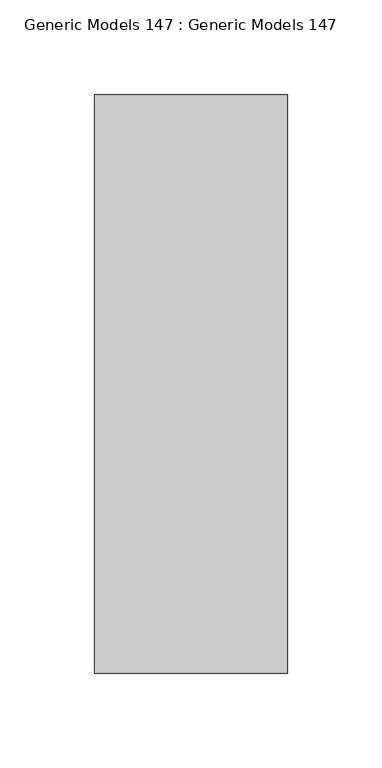
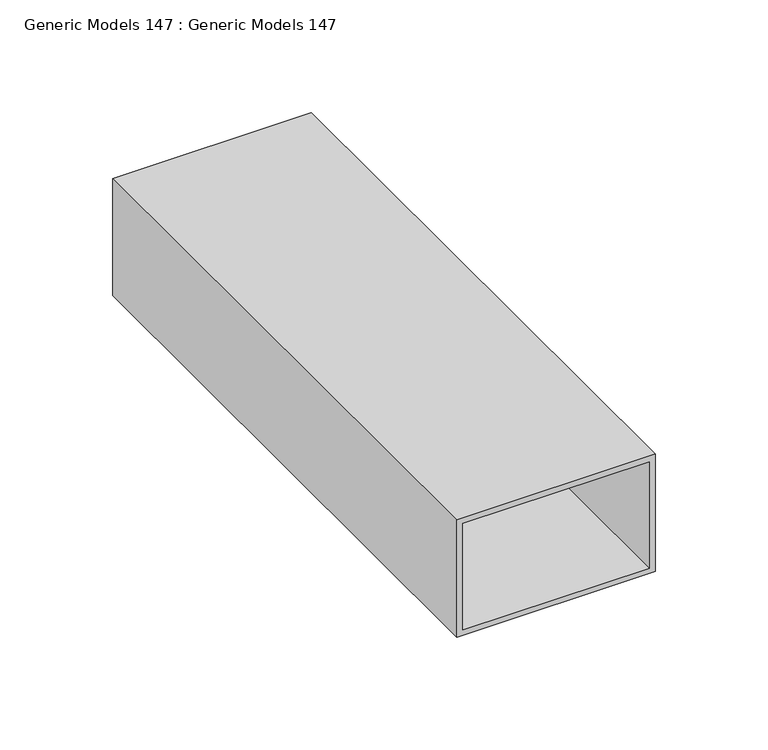
"""IFC4 building model written with IfcOpenShell, lengths in millimetres: proxy geometry, Generic Models 147 : Generic Models 147."""

from ifc_helpers import new_model, si_unit, frame, origin, place, context, project, spatial, polyline, outline, extrude, source, transform, mapped, element, save


def generic_models_147_generic_models_147_e6257d2f(model_context):
    return source(origin(), model_context, "Body", "SweptSolid", [
        extrude(outline(polyline([(126263.146, 4942.0939304), (126263.146, 4840.4939304), (126199.646, 4840.4939304), (126199.646, 4942.0939304), (126263.146, 4942.0939304)]), holes=[polyline([(126260.0346675, 4939.0291173), (126202.4292591, 4939.0291173), (126202.4292591, 4843.5123667), (126260.0346675, 4843.5123667), (126260.0346675, 4939.0291173)])]), frame((0.0, 399.7309662, 0.0), z_axis=(0.0, 1.0, 0.0), x_axis=(0.0, 0.0, 1.0)), (0.0, 0.0, 1.0), 304.8),
    ])


if __name__ == "__main__":
    model = new_model("IFC4")
    model_context = context("Model", 3, world=origin())
    ifc_project = project(units=[si_unit("LENGTHUNIT", "METRE", prefix="MILLI")], contexts=[model_context])
    site = spatial("IfcSite", under=ifc_project)
    building = spatial("IfcBuilding", under=site)
    placement = place(None, origin())
    generic_models_147_generic_models_147_shape = generic_models_147_generic_models_147_e6257d2f(model_context)
    element("IfcBuildingElementProxy", 1, Name="Generic Models 147 : Generic Models 147", ObjectType="Generic Models 147 : Generic Models 147", at=placement, inside=building, context=model_context, shape_type="MappedRepresentation", body=[
        mapped(generic_models_147_generic_models_147_shape, transform((0.0, 0.0, 0.0), x_axis=(1.0, 0.0, 0.0), y_axis=(0.0, 1.0, 0.0), z_axis=(0.0, 0.0, 1.0))),
    ])
    save(model, "model.ifc")

# Revit data of these elements
# Element 1 (IfcBuildingElementProxy, "Generic Models 147 : Generic Models 147")
#   Materials on its faces: "_STRUCTURAL STEEL (SEE STRUCT. DWGS)"
# Materials
#   "_STRUCTURAL STEEL (SEE STRUCT. DWGS)": class "Metal", colour RGB 199 199 199, transparency 0, Description = "Structural steel 50ksi", Cost = 0
